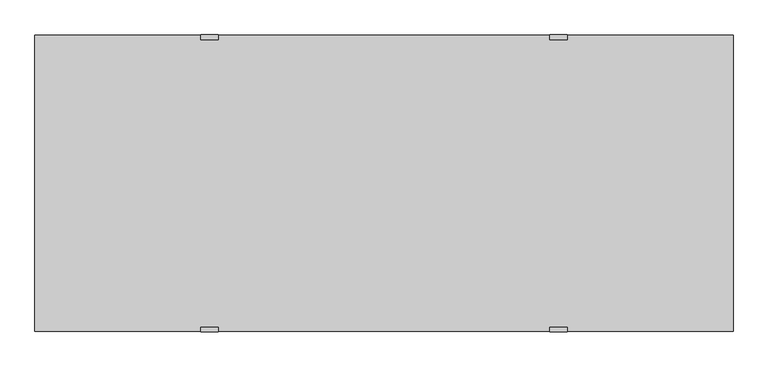
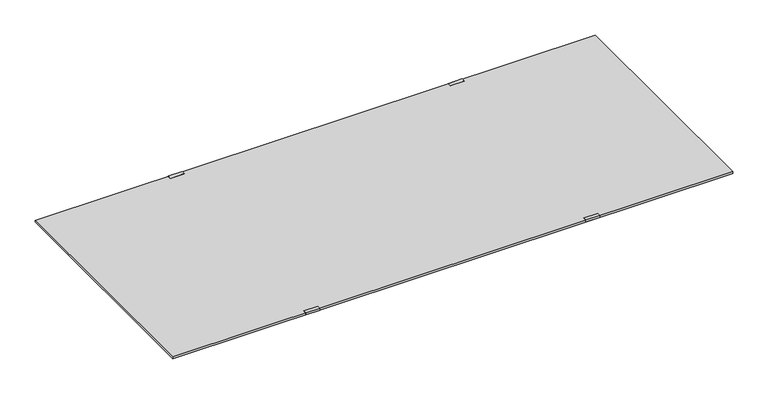
"""IFC4 building model written with IfcOpenShell, lengths in millimetres: proxy geometry."""

from ifc_helpers import new_model, si_unit, frame, origin, origin_with_axes, place, context, project, spatial, polyline, outline, extrude, source, transform, mapped, element, save


def specialty_equipment_f3c8ae46(model_context):
    return source(origin(), model_context, "Body", "SweptSolid", [
        extrude(outline(polyline([(-431.8, 6.35), (-431.8, 0.0), (-432.59375, 0.0), (-432.59375, 7.14375), (-419.1, 7.14375), (-419.1, 6.35), (-431.8, 6.35)])), frame((482.6, 0.0, 0.0), z_axis=(1.0, 0.0, 0.0), x_axis=(0.0, 1.0, 0.0)), (0.0, 0.0, 1.0), 50.8),
        extrude(outline(polyline([(-431.8, 6.35), (-431.8, 0.0), (-432.59375, 0.0), (-432.59375, 7.14375), (-419.1, 7.14375), (-419.1, 6.35), (-431.8, 6.35)])), frame((-533.4, 0.0, 0.0), z_axis=(1.0, 0.0, 0.0), x_axis=(0.0, 1.0, 0.0)), (0.0, 0.0, 1.0), 50.8),
        extrude(outline(polyline([(431.8, 6.35), (419.1, 6.35), (419.1, 7.14375), (432.59375, 7.14375), (432.59375, 0.0), (431.8, 0.0), (431.8, 6.35)])), frame((482.6, 0.0, 0.0), z_axis=(1.0, 0.0, 0.0), x_axis=(0.0, 1.0, 0.0)), (0.0, 0.0, 1.0), 50.8),
        extrude(outline(polyline([(431.8, 6.35), (419.1, 6.35), (419.1, 7.14375), (432.59375, 7.14375), (432.59375, 0.0), (431.8, 0.0), (431.8, 6.35)])), frame((-533.4, 0.0, 0.0), z_axis=(1.0, 0.0, 0.0), x_axis=(0.0, 1.0, 0.0)), (0.0, 0.0, 1.0), 50.8),
        extrude(outline(polyline([(1016.0, 431.8), (1016.0, -431.8), (-1016.0, -431.8), (-1016.0, 431.8), (1016.0, 431.8)])), origin_with_axes(), (0.0, 0.0, 1.0), 6.35),
    ])


if __name__ == "__main__":
    model = new_model("IFC4")
    model_context = context("Model", 3, world=origin())
    ifc_project = project(units=[si_unit("LENGTHUNIT", "METRE", prefix="MILLI")], contexts=[model_context])
    site = spatial("IfcSite", under=ifc_project)
    building = spatial("IfcBuilding", under=site)
    placement = place(None, origin())
    specialty_equipment_shape = specialty_equipment_f3c8ae46(model_context)
    element("IfcBuildingElementProxy", 1, Name="Bradley-Washroom_Accessories-Mirrors-747_Standard : 60\" x 36\" + BradEX", ObjectType="Bradley-Washroom_Accessories-Mirrors-747_Standard : 60\" x 36\" + BradEX", at=placement, inside=building, context=model_context, shape_type="MappedRepresentation", body=[
        mapped(specialty_equipment_shape, transform((0.0, 0.0, 0.0), x_axis=(1.0, 0.0, 0.0), y_axis=(0.0, 1.0, 0.0), z_axis=(0.0, 0.0, 1.0))),
    ])
    save(model, "model.ifc")

# Revit data of these elements
# Type "Bradley-Washroom_Accessories-Mirrors-747_Standard : 60\" x 36\" + BradEX"
#   Keynote = "M08831300.01"
#   Warranty Information = "Complete unit, excepting mirrors warranted for one year.\r\n Stainless steel mirror frames for fifteen years.\r\n Plate glass mirrors for fifteen years.\r\n This warranty does not cover installation or any other labor charges and does not apply to any units,\r\n which have been damaged by accident, abuse, improper installation, improper maintenance, or altered in any way."
#   Version = "1.0"
#   URL = "http://www.bradleycorp.com/"
#   Type Comments = "BradEX 1/4\" Float Glass Mirror"
#   OmniClass Title = "Mirrors"
#   OmniClass Code = "23.40.95.17.17"
#   Modeling Code = ""
#   Model = "747-024360"
#   MasterFormat Title = "Commercial Toilet Accessories"
#   MasterFormat Number = "10 28 13. 13"
#   Manufacturer = "Bradley Corporation"
#   Industry Standards = "ASTM C 1036"
#   Fire Rating = "n/a"
#   Description = "Frameless Mirror, Clip Fasteners, 24 by 36 inches"
#   Copyright = "This Model Data is Property of Bradley Corporation"
#   Buy American Act = "Yes"
#   Assembly Code = "C1030900"
#   ADA Compliant = "Yes"
#   Width = 6' - 8"
#   Height = 2' - 10"
#   Fastener Placement = 1' - 8"
#   Depth = 0' - 0 1/4"
#   Default Elevation = 3' - 4"
#   Reflective Material = Glass - Bradley Corp - BradEX - Polished Float Mirror
#   Frame Material = Bradley Corp Stainless Steel - Satin
# Element 1 (IfcBuildingElementProxy, "Bradley-Washroom_Accessories-Mirrors-747_Standard : 60\" x 36\" + BradEX")
#   Materials on its faces: "Bradley Corp Stainless Steel - Satin", "Glass - Bradley Corp - BradEX - Polished Float Mirror"
# Materials
#   "Glass - Bradley Corp - BradEX - Polished Float Mirror": class "Glass", colour RGB 221 230 232, transparency 0, Manufacturer = "Bradley Corporation", URL = "www.bradleycorp.com", Description = "Stainless Steel - Satin Finish", Cost = 0
#   "Bradley Corp Stainless Steel - Satin": class "Metal", colour RGB 189 187 185, transparency 0, Manufacturer = "Bradley Corporation", URL = "www.bradleycorp.com", Description = "Stainless Steel - Satin Finish", Cost = 0
